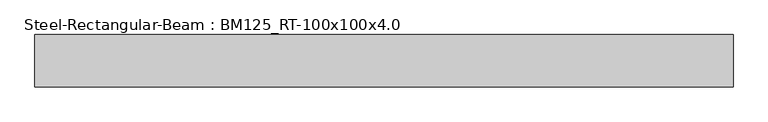
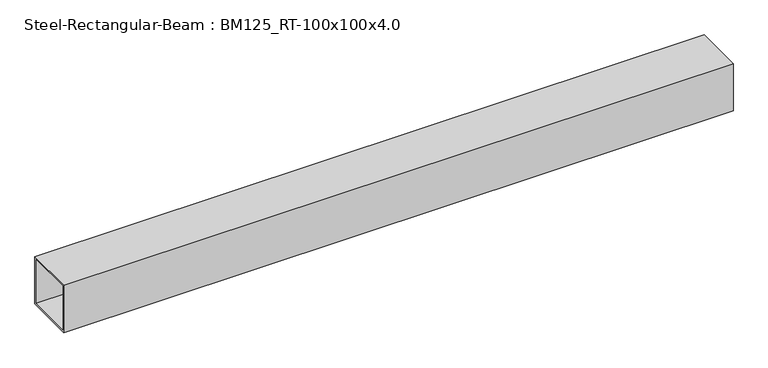
"""IFC4 building model written with IfcOpenShell, lengths in millimetres: beam geometry, Steel-Rectangular-Beam : BM125_RT-100x100x4.0."""

import ifcopenshell
import ifcopenshell.guid

model = None  # the IFC model being written
_history = None  # IfcOwnerHistory: only IFC2X3 demands one
_inside = {}  # id of a spatial element -> (the spatial element, [elements in it])
_under = {}  # id of a project, library or spatial element -> (it, [spatial elements below it])
_declared = {}  # id of a project -> (the project, [libraries it declares])
_typed = {}  # id of a type object -> (the type object, [elements of that type])
_made_of = {}  # id of a material, layer set ... -> (it, [elements and type objects made of it])


def new_model(schema):
    """Start an empty IFC model of exactly this schema.

    Asked for "IFC4X3", IfcOpenShell would pick the latest addendum, in which some entities
    have other attributes; the version numbers below select the first issue.
    IFC2X3 requires an IfcOwnerHistory on every rooted entity: one is made here for all.
    """
    global model, _history
    if schema == "IFC4X3":
        model = ifcopenshell.file(schema_version=(4, 3, 0, 0))
    else:
        model = ifcopenshell.file(schema=schema)
    _inside.clear()
    _under.clear()
    _declared.clear()
    _typed.clear()
    _made_of.clear()
    _history = None
    if model.schema == "IFC2X3":
        org = make("IfcOrganization", Name="unknown")
        user = make(
            "IfcPersonAndOrganization",
            ThePerson=make("IfcPerson", FamilyName="unknown"),
            TheOrganization=org,
        )
        app = make(
            "IfcApplication",
            ApplicationDeveloper=org,
            Version="unknown",
            ApplicationFullName="unknown",
            ApplicationIdentifier="unknown",
        )
        _history = make(
            "IfcOwnerHistory",
            OwningUser=user,
            OwningApplication=app,
            ChangeAction="ADDED",
            CreationDate=0,
        )
    return model


def make(cls, **values):
    """One entity of the class cls with the attributes given. An attribute that is None is left unset."""
    return model.create_entity(
        cls, **{name: value for name, value in values.items() if value is not None}
    )


def rooted(cls, **values):
    """An entity with a GlobalId (a new one), such as an element, a storey or a relation."""
    return make(cls, GlobalId=ifcopenshell.guid.new(), OwnerHistory=_history, **values)


def si_unit(unit_type, name, prefix=None):
    """IfcSIUnit, for example si_unit("LENGTHUNIT", "METRE", prefix="MILLI")."""
    return make("IfcSIUnit", UnitType=unit_type, Prefix=prefix, Name=name)


def assignment(units):
    """IfcUnitAssignment: the units of a project."""
    return None if units is None else make("IfcUnitAssignment", Units=units)


def point(xyz):
    """IfcCartesianPoint."""
    return None if xyz is None else make("IfcCartesianPoint", Coordinates=xyz)


def direction(xyz):
    """IfcDirection."""
    return None if xyz is None else make("IfcDirection", DirectionRatios=xyz)


def frame(location, z_axis=None, x_axis=None):
    """IfcAxis2Placement3D, a coordinate frame: its origin and axes. An axis left out is left unset."""
    return make(
        "IfcAxis2Placement3D",
        Location=point(location),
        Axis=direction(z_axis),
        RefDirection=direction(x_axis),
    )


def origin():
    """The frame at (0, 0, 0) with its axes left unset."""
    return frame((0.0, 0.0, 0.0))


def place(relative_to, where):
    """IfcLocalPlacement: puts the frame where relative to a parent placement (None: the world)."""
    return make(
        "IfcLocalPlacement", PlacementRelTo=relative_to, RelativePlacement=where
    )


def context(
    kind, dimensions, precision=None, world=None, true_north=None, identifier=None
):
    """IfcGeometricRepresentationContext, for example the 3D "Model" context."""
    return make(
        "IfcGeometricRepresentationContext",
        ContextIdentifier=identifier,
        ContextType=kind,
        CoordinateSpaceDimension=dimensions,
        Precision=precision,
        WorldCoordinateSystem=world,
        TrueNorth=true_north,
    )


def project(units=None, contexts=None):
    """IfcProject with its units and contexts."""
    return rooted(
        "IfcProject",
        Name="project",
        RepresentationContexts=contexts,
        UnitsInContext=assignment(units),
    )


def spatial(cls, under=None, at=None, **own):
    """A site, building, storey or space (cls), placed at a placement, below another one or the project."""
    s = rooted(cls, ObjectPlacement=at, **own)
    if under is not None:
        _under.setdefault(under.id(), (under, []))[1].append(s)
    return s


def polyline(points):
    """IfcPolyline through the points."""
    return make("IfcPolyline", Points=[point(p) for p in points])


def outline(outer, holes=None, kind="AREA"):
    """IfcArbitraryClosedProfileDef: a profile drawn as a closed curve; with holes, ...WithVoids."""
    if holes is None:
        return make("IfcArbitraryClosedProfileDef", ProfileType=kind, OuterCurve=outer)
    return make(
        "IfcArbitraryProfileDefWithVoids",
        ProfileType=kind,
        OuterCurve=outer,
        InnerCurves=holes,
    )


def extrude(swept, where, along, depth):
    """IfcExtrudedAreaSolid: the profile swept, set in the frame where, extruded along a direction by depth."""
    return make(
        "IfcExtrudedAreaSolid",
        SweptArea=swept,
        Position=where,
        ExtrudedDirection=direction(along),
        Depth=depth,
    )


def shape(context_of_items, identifier, shape_type, items):
    """IfcShapeRepresentation: the items that make up one representation, for example the "Body"."""
    return make(
        "IfcShapeRepresentation",
        ContextOfItems=context_of_items,
        RepresentationIdentifier=identifier,
        RepresentationType=shape_type,
        Items=items,
    )


def source(mapping_origin, context_of_items, identifier, shape_type, items):
    """IfcRepresentationMap: a shape defined once, which mapped items show again and again."""
    return make(
        "IfcRepresentationMap",
        MappingOrigin=mapping_origin,
        MappedRepresentation=shape(context_of_items, identifier, shape_type, items),
    )


def transform(
    local_origin,
    x_axis=None,
    y_axis=None,
    z_axis=None,
    scale=None,
    scale2=None,
    scale3=None,
    uniform=True,
):
    """IfcCartesianTransformationOperator3D, or its non-uniform kind. x_axis, y_axis, z_axis: its Axis1, 2, 3."""
    if uniform:
        return make(
            "IfcCartesianTransformationOperator3D",
            Axis1=direction(x_axis),
            Axis2=direction(y_axis),
            LocalOrigin=point(local_origin),
            Scale=scale,
            Axis3=direction(z_axis),
        )
    return make(
        "IfcCartesianTransformationOperator3DnonUniform",
        Axis1=direction(x_axis),
        Axis2=direction(y_axis),
        LocalOrigin=point(local_origin),
        Scale=scale,
        Axis3=direction(z_axis),
        Scale2=scale2,
        Scale3=scale3,
    )


def mapped(mapping_source, mapping_target):
    """IfcMappedItem: shows the shape of a source again, moved by a transform."""
    return make(
        "IfcMappedItem", MappingSource=mapping_source, MappingTarget=mapping_target
    )


def made_of(thing, what):
    """Note that an element or type object is made of a material, layer set ...; save() writes the relation."""
    if what is not None:
        _made_of.setdefault(what.id(), (what, []))[1].append(thing)
    return thing


def element(
    cls,
    number,
    at=None,
    inside=None,
    cuts=None,
    type_object=None,
    material=None,
    context=None,
    identifier="Body",
    shape_type=None,
    held_by="IfcProductDefinitionShape",
    body=None,
    shapes=None,
    **own,
):
    """One element of the class cls, such as IfcWall. Its Tag is "e" and its number.

    at: its placement. inside: the storey or other place that contains it. cuts: it is an
    opening in that element (IfcRelVoidsElement). A single representation is given by context,
    identifier, shape_type and body (its items); several are given by shapes. held_by: the class
    of the entity that holds the representations. save() writes the other relations.
    """
    e = rooted(cls, Tag="e%d" % number, ObjectPlacement=at, **own)
    if body is not None:
        shapes = [shape(context, identifier, shape_type, body)]
    if shapes is not None:
        e.Representation = make(held_by, Representations=shapes)
    if inside is not None:
        _inside.setdefault(inside.id(), (inside, []))[1].append(e)
    if cuts is not None:
        rooted(
            "IfcRelVoidsElement", RelatingBuildingElement=cuts, RelatedOpeningElement=e
        )
    if type_object is not None:
        _typed.setdefault(type_object.id(), (type_object, []))[1].append(e)
    return made_of(e, material)


def aggregate(whole, parts):
    """IfcRelAggregates: a whole, such as a stair, and the parts it consists of."""
    return rooted("IfcRelAggregates", RelatingObject=whole, RelatedObjects=parts)


def save(model, path):
    """Write the relations noted so far, then the file.

    IfcRelAggregates (storeys below a building ...), IfcRelContainedInSpatialStructure (elements
    in a storey), IfcRelDefinesByType, IfcRelAssociatesMaterial and IfcRelDeclares: one each for
    every whole, place, type object, material and project.
    """
    for whole, parts in _under.values():
        aggregate(whole, parts)
    for where, things in _inside.values():
        rooted(
            "IfcRelContainedInSpatialStructure",
            RelatedElements=things,
            RelatingStructure=where,
        )
    for kind, things in _typed.values():
        rooted("IfcRelDefinesByType", RelatedObjects=things, RelatingType=kind)
    for what, things in _made_of.values():
        rooted("IfcRelAssociatesMaterial", RelatedObjects=things, RelatingMaterial=what)
    for by, libraries in _declared.values():
        rooted("IfcRelDeclares", RelatingContext=by, RelatedDefinitions=libraries)
    model.write(path)


def steel_rectangular_beam_bm125_rt_100x100x4_0_d4cde651(model_context):
    return source(origin(), model_context, "Body", "SweptSolid", [
        extrude(outline(polyline([(-50.0, 50.0), (50.0, 50.0), (50.0, -50.0), (-50.0, -50.0), (-50.0, 50.0)]), holes=[polyline([(46.0, -46.0), (46.0, 46.0), (-46.0, 46.0), (-46.0, -46.0), (46.0, -46.0)])]), frame((-612.3, 0.0, 0.0), z_axis=(1.0, 0.0, 0.0), x_axis=(0.0, 1.0, 0.0)), (0.0, 0.0, 1.0), 1337.3),
        extrude(outline(polyline([(-50.0, 50.0), (50.0, 50.0), (50.0, -50.0), (-50.0, -50.0), (-50.0, 50.0)]), holes=[polyline([(46.0, -46.0), (46.0, 46.0), (-46.0, 46.0), (-46.0, -46.0), (46.0, -46.0)])]), frame((-612.3, 0.0, 0.0), z_axis=(1.0, 0.0, 0.0), x_axis=(0.0, 1.0, 0.0)), (0.0, 0.0, 1.0), 1337.3),
        extrude(outline(polyline([(-50.0, 50.0), (50.0, 50.0), (50.0, -50.0), (-50.0, -50.0), (-50.0, 50.0)]), holes=[polyline([(46.0, -46.0), (46.0, 46.0), (-46.0, 46.0), (-46.0, -46.0), (46.0, -46.0)])]), frame((-612.3, 0.0, 0.0), z_axis=(1.0, 0.0, 0.0), x_axis=(0.0, 1.0, 0.0)), (0.0, 0.0, 1.0), 1337.3),
        extrude(outline(polyline([(-50.0, 50.0), (50.0, 50.0), (50.0, -50.0), (-50.0, -50.0), (-50.0, 50.0)]), holes=[polyline([(46.0, -46.0), (46.0, 46.0), (-46.0, 46.0), (-46.0, -46.0), (46.0, -46.0)])]), frame((-612.3, 0.0, 0.0), z_axis=(1.0, 0.0, 0.0), x_axis=(0.0, 1.0, 0.0)), (0.0, 0.0, 1.0), 1337.3),
    ])


if __name__ == "__main__":
    model = new_model("IFC4")
    model_context = context("Model", 3, world=origin())
    ifc_project = project(units=[si_unit("LENGTHUNIT", "METRE", prefix="MILLI")], contexts=[model_context])
    site = spatial("IfcSite", under=ifc_project)
    building = spatial("IfcBuilding", under=site)
    placement = place(None, origin())
    steel_rectangular_beam_bm125_rt_100x100x4_0_shape = steel_rectangular_beam_bm125_rt_100x100x4_0_d4cde651(model_context)
    element("IfcBeam", 1, ObjectType="Steel-Rectangular-Beam : BM125_RT-100x100x4.0", at=placement, inside=building, context=model_context, shape_type="MappedRepresentation", body=[
        mapped(steel_rectangular_beam_bm125_rt_100x100x4_0_shape, transform((0.0, 0.0, 0.0), x_axis=(1.0, 0.0, 0.0), y_axis=(0.0, 1.0, 0.0), z_axis=(0.0, 0.0, 1.0))),
    ])
    save(model, "model.ifc")

# Revit data of these elements
# Type "Steel-Rectangular-Beam : BM125_RT-100x100x4.0"
#   t = 4 mm
#   Mass per Unit Length = 11.70 kg/m
#   Surface Area = 0.386 m²/m
#   Sectional Area = 14.95 cm²
#   Length [instance default] = 3000 mm
#   H = 100 mm
#   B = 100 mm
#   hec_material4 [instance default] = none
#   hec_material3 [instance default] = none
#   hec_material2 [instance default] = none
#   hec_material1 [instance default] = none
#   Structural Material [instance default] = none
# Element 1 (IfcBeam, "Steel-Rectangular-Beam : BM125_RT-100x100x4.0")
#   hec_material2 = S01AA010-00001_Main Steel Structure Fabrication Work_Shelter/Building_Steel Painting/Coating_for Non-Fireproofed Steel Surface, Surface Preparation, Primer, Second & Final Coat
#   hec_material1 = S03AA007-00001_Main Steel Structure Erection Work_Girth & Purlin
#   Structural Material = S01AA007-00001_Main Steel Structure Fabrication Work_Shelter/Building_Girth & Purlin
#   Materials on its faces: "S01AA010-00001_Main Steel Structure Fabrication Work_Shelter/Building_Steel Painting/Coating_for Non-Fireproofed Steel Surface, Surface Preparation, Primer, Second & Final Coat"
# Materials
#   "S01AA010-00001_Main Steel Structure Fabrication Work_Shelter/Building_Steel Painting/Coating_for Non-Fireproofed Steel Surface, Surface Preparation, Primer, Second & Final Coat": class "Metal", colour RGB 120 120 120, transparency 0, Description = "Paint finished steel", W00) Work Master Code = "S01AA010-00001", W01) Work Master_Lv1 = "Main Steel Structure Fabrication Work", W02) Work Master_Lv2 = "Shelter/Building", W03) Work Master_Spec.1 = "Steel Painting/Coating", W04) Work Master_Spec.2 = "for Non-Fireproofed Steel Surface, Surface Preparation, Primer, Second & Final Coat", Cost = 0
#   "S03AA007-00001_Main Steel Structure Erection Work_Girth & Purlin": class "Metal", colour RGB 120 120 120, transparency 0, Comments = "(30KG/M>Weight)", Description = "Structural steel 50ksi", W00) Work Master Code = "S03AA007-00001", W01) Work Master_Lv1 = "Main Steel Structure Erection Work", W02) Work Master_Lv2 = "Shelter/Building", W03) Work Master_Spec.1 = "Girth & Purlin", Cost = 0
#   "S01AA007-00001_Main Steel Structure Fabrication Work_Shelter/Building_Girth & Purlin": class "Metal", colour RGB 120 120 120, transparency 0, Comments = "(30KG/M>Weight)", Description = "Structural steel 50ksi", W00) Work Master Code = "S01AA007-00001", W01) Work Master_Lv1 = "Main Steel Structure Fabrication Work", W02) Work Master_Lv2 = "Shelter/Building", W03) Work Master_Spec.1 = "Girth & Purlin", Cost = 0
